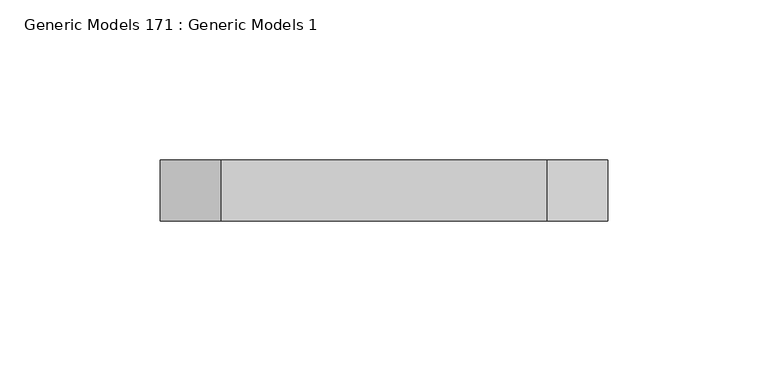
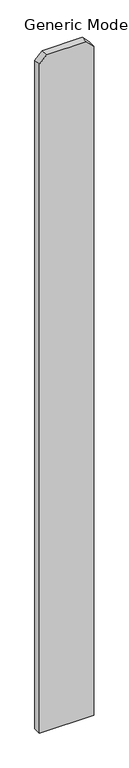
"""IFC4 building model written with IfcOpenShell, lengths in millimetres: proxy geometry, Generic Models 171 : Generic Models 1."""

from ifc_helpers import new_model, si_unit, frame, origin, place, context, project, spatial, polyline, outline, extrude, source, transform, mapped, element, save


def generic_models_171_generic_models_1_1e9a53e4(model_context):
    return source(origin(), model_context, "Body", "SweptSolid", [
        extrude(outline(polyline([(76.2, 56056.2125), (1885.95, 56056.2125), (1905.0, 56037.1625), (1905.0, 55935.5625), (1885.95, 55916.5125), (76.2, 55916.5125), (76.2, 56056.2125)])), frame((0.0, 547.6875, 0.0), z_axis=(0.0, 1.0, 0.0), x_axis=(0.0, 0.0, 1.0)), (0.0, 0.0, 1.0), 19.05),
    ])


if __name__ == "__main__":
    model = new_model("IFC4")
    model_context = context("Model", 3, world=origin())
    ifc_project = project(units=[si_unit("LENGTHUNIT", "METRE", prefix="MILLI")], contexts=[model_context])
    site = spatial("IfcSite", under=ifc_project)
    building = spatial("IfcBuilding", under=site)
    placement = place(None, origin())
    generic_models_171_generic_models_1_shape = generic_models_171_generic_models_1_1e9a53e4(model_context)
    element("IfcBuildingElementProxy", 1, Name="Generic Models 171 : Generic Models 1", ObjectType="Generic Models 171 : Generic Models 1", at=placement, inside=building, context=model_context, shape_type="MappedRepresentation", body=[
        mapped(generic_models_171_generic_models_1_shape, transform((0.0, 0.0, 0.0), x_axis=(1.0, 0.0, 0.0), y_axis=(0.0, 1.0, 0.0), z_axis=(0.0, 0.0, 1.0))),
    ])
    save(model, "model.ifc")

# Revit data of these elements
# Element 1 (IfcBuildingElementProxy, "Generic Models 171 : Generic Models 1")
#   Materials on its faces: "VERTICAL 1X6 CEDAR PLANKS W/ CLEAR WOOD SEALER"
# Materials
#   "VERTICAL 1X6 CEDAR PLANKS W/ CLEAR WOOD SEALER": class "Wood", colour RGB 234 198 147, transparency 0, Description = "Pinus Echinata", Cost = 0
